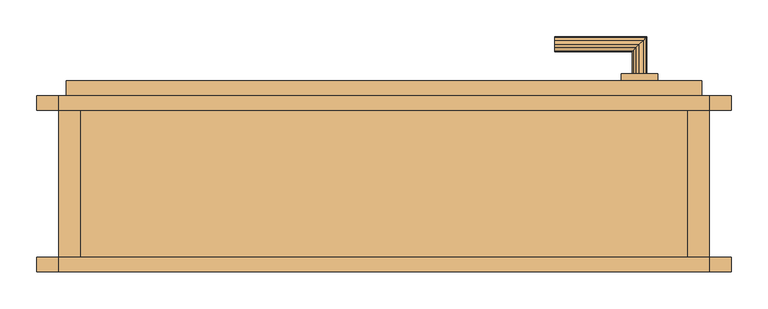
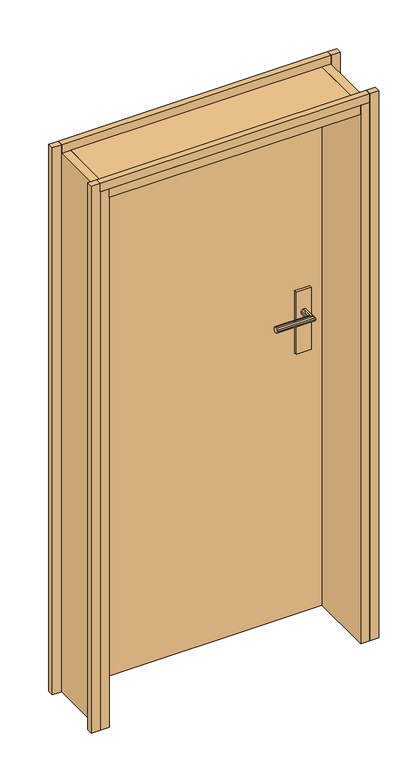
"""IFC4 building model written with IfcOpenShell, lengths in millimetres: door geometry, Tür."""

from ifc_helpers import new_model, si_unit, frame, origin, place, context, project, spatial, polyline, outline, extrude, faceted_brep, source, transform, mapped, element, save


def door_08fc6649(model_context):
    return source(origin(), model_context, "Body", "SolidModel", [
        extrude(outline(polyline([(885.0, 0.0), (885.0, -20.0), (0.0, -20.0), (0.0, 0.0), (885.0, 0.0)])), frame((0.0, 0.0, 2010.0), z_axis=(0.0, 0.0, 1.0), x_axis=(1.0, 0.0, 0.0)), (0.0, 0.0, 1.0), 30.0),
        extrude(outline(polyline([(815.0, 250.0), (815.0, 240.0), (765.0, 240.0), (765.0, 250.0), (815.0, 250.0)])), frame((0.0, 0.0, 1050.0), z_axis=(0.0, 0.0, 1.0), x_axis=(1.0, 0.0, 0.0)), (0.0, 0.0, 1.0), 215.0),
        extrude(outline(polyline([(915.0, 0.0), (915.0, -20.0), (885.0, -20.0), (885.0, 0.0), (915.0, 0.0)])), frame((0.0, 0.0, 140.0), z_axis=(0.0, 0.0, 1.0), x_axis=(1.0, 0.0, 0.0)), (0.0, 0.0, 1.0), 1900.0),
        extrude(outline(polyline([(855.0, 220.0), (855.0, -20.0), (30.0, -20.0), (30.0, 220.0), (855.0, 220.0)])), frame((0.0, 0.0, 1980.0), z_axis=(0.0, 0.0, 1.0), x_axis=(1.0, 0.0, 0.0)), (0.0, 0.0, 1.0), 30.0),
        extrude(outline(polyline([(0.0, -20.0), (-30.0, -20.0), (-30.0, 0.0), (0.0, 0.0), (0.0, -20.0)])), frame((0.0, 0.0, 140.0), z_axis=(0.0, 0.0, 1.0), x_axis=(1.0, 0.0, 0.0)), (0.0, 0.0, 1.0), 1900.0),
        extrude(outline(polyline([(765.0, 200.0), (815.0, 200.0), (815.0, 190.0), (765.0, 190.0), (765.0, 200.0)])), frame((0.0, 0.0, 1050.0), z_axis=(0.0, 0.0, 1.0), x_axis=(1.0, 0.0, 0.0)), (0.0, 0.0, 1.0), 215.0),
        extrude(outline(polyline([(885.0, 220.0), (885.0, -20.0), (855.0, -20.0), (855.0, 220.0), (885.0, 220.0)])), frame((0.0, 0.0, 140.0), z_axis=(0.0, 0.0, 1.0), x_axis=(1.0, 0.0, 0.0)), (0.0, 0.0, 1.0), 1870.0),
        faceted_brep([(795.0, 250.0, 1198.660254), (790.0, 250.0, 1200.0), (785.0, 250.0, 1198.660254), (781.339746, 250.0, 1195.0), (780.0, 250.0, 1190.0), (781.339746, 250.0, 1185.0), (785.0, 250.0, 1181.339746), (790.0, 250.0, 1180.0), (795.0, 250.0, 1181.339746), (798.660254, 250.0, 1185.0), (800.0, 250.0, 1190.0), (798.660254, 250.0, 1195.0), (790.0, 290.0, 1200.0), (795.0, 295.0, 1198.660254), (798.660254, 298.660254, 1195.0), (800.0, 300.0, 1190.0), (798.660254, 298.660254, 1185.0), (795.0, 295.0, 1181.339746), (790.0, 290.0, 1180.0), (785.0, 285.0, 1181.339746), (781.339746, 281.339746, 1185.0), (780.0, 280.0, 1190.0), (781.339746, 281.339746, 1195.0), (785.0, 285.0, 1198.660254), (675.0, 285.0, 1198.660254), (675.0, 290.0, 1200.0), (675.0, 295.0, 1198.660254), (675.0, 298.660254, 1195.0), (675.0, 300.0, 1190.0), (675.0, 298.660254, 1185.0), (675.0, 295.0, 1181.339746), (675.0, 290.0, 1180.0), (675.0, 285.0, 1181.339746), (675.0, 281.339746, 1185.0), (675.0, 280.0, 1190.0), (675.0, 281.339746, 1195.0)], [[[0, 1, 2, 3, 4, 5, 6, 7, 8, 9, 10, 11]], [[12, 1, 0, 13]], [[13, 0, 11, 14]], [[14, 11, 10, 15]], [[15, 10, 9, 16]], [[16, 9, 8, 17]], [[17, 8, 7, 18]], [[18, 7, 6, 19]], [[19, 6, 5, 20]], [[20, 5, 4, 21]], [[21, 4, 3, 22]], [[22, 3, 2, 23]], [[23, 2, 1, 12]], [[24, 25, 26, 27, 28, 29, 30, 31, 32, 33, 34, 35]], [[25, 12, 13, 26]], [[26, 13, 14, 27]], [[27, 14, 15, 28]], [[28, 15, 16, 29]], [[29, 16, 17, 30]], [[30, 17, 18, 31]], [[31, 18, 19, 32]], [[32, 19, 20, 33]], [[33, 20, 21, 34]], [[34, 21, 22, 35]], [[35, 22, 23, 24]], [[24, 23, 12, 25]]]),
        extrude(outline(polyline([(885.0, 220.0), (885.0, 200.0), (0.0, 200.0), (0.0, 220.0), (885.0, 220.0)])), frame((0.0, 0.0, 2010.0), z_axis=(0.0, 0.0, 1.0), x_axis=(1.0, 0.0, 0.0)), (0.0, 0.0, 1.0), 30.0),
        extrude(outline(polyline([(875.0, 240.0), (875.0, 200.0), (10.0, 200.0), (10.0, 240.0), (875.0, 240.0)])), frame((0.0, 0.0, 140.0), z_axis=(0.0, 0.0, 1.0), x_axis=(1.0, 0.0, 0.0)), (0.0, 0.0, 1.0), 1860.0),
        extrude(outline(polyline([(0.0, 200.0), (-30.0, 200.0), (-30.0, 220.0), (0.0, 220.0), (0.0, 200.0)])), frame((0.0, 0.0, 140.0), z_axis=(0.0, 0.0, 1.0), x_axis=(1.0, 0.0, 0.0)), (0.0, 0.0, 1.0), 1900.0),
        faceted_brep([(785.0, 190.0, 1198.660254), (790.0, 190.0, 1200.0), (795.0, 190.0, 1198.660254), (798.660254, 190.0, 1195.0), (800.0, 190.0, 1190.0), (798.660254, 190.0, 1185.0), (795.0, 190.0, 1181.339746), (790.0, 190.0, 1180.0), (785.0, 190.0, 1181.339746), (781.339746, 190.0, 1185.0), (780.0, 190.0, 1190.0), (781.339746, 190.0, 1195.0), (790.0, 150.0, 1200.0), (795.0, 145.0, 1198.660254), (798.660254, 141.339746, 1195.0), (800.0, 140.0, 1190.0), (798.660254, 141.339746, 1185.0), (795.0, 145.0, 1181.339746), (790.0, 150.0, 1180.0), (785.0, 155.0, 1181.339746), (781.339746, 158.660254, 1185.0), (780.0, 160.0, 1190.0), (781.339746, 158.660254, 1195.0), (785.0, 155.0, 1198.660254), (675.0, 145.0, 1198.660254), (675.0, 150.0, 1200.0), (675.0, 155.0, 1198.660254), (675.0, 158.660254, 1195.0), (675.0, 160.0, 1190.0), (675.0, 158.660254, 1185.0), (675.0, 155.0, 1181.339746), (675.0, 150.0, 1180.0), (675.0, 145.0, 1181.339746), (675.0, 141.339746, 1185.0), (675.0, 140.0, 1190.0), (675.0, 141.339746, 1195.0)], [[[0, 1, 2, 3, 4, 5, 6, 7, 8, 9, 10, 11]], [[2, 1, 12, 13]], [[3, 2, 13, 14]], [[4, 3, 14, 15]], [[5, 4, 15, 16]], [[6, 5, 16, 17]], [[7, 6, 17, 18]], [[8, 7, 18, 19]], [[9, 8, 19, 20]], [[10, 9, 20, 21]], [[11, 10, 21, 22]], [[0, 11, 22, 23]], [[1, 0, 23, 12]], [[24, 25, 26, 27, 28, 29, 30, 31, 32, 33, 34, 35]], [[13, 12, 25, 24]], [[14, 13, 24, 35]], [[15, 14, 35, 34]], [[16, 15, 34, 33]], [[17, 16, 33, 32]], [[18, 17, 32, 31]], [[19, 18, 31, 30]], [[20, 19, 30, 29]], [[21, 20, 29, 28]], [[22, 21, 28, 27]], [[23, 22, 27, 26]], [[12, 23, 26, 25]]]),
        extrude(outline(polyline([(915.0, 220.0), (915.0, 200.0), (885.0, 200.0), (885.0, 220.0), (915.0, 220.0)])), frame((0.0, 0.0, 140.0), z_axis=(0.0, 0.0, 1.0), x_axis=(1.0, 0.0, 0.0)), (0.0, 0.0, 1.0), 1900.0),
        extrude(outline(polyline([(30.0, 220.0), (30.0, -20.0), (0.0, -20.0), (0.0, 220.0), (30.0, 220.0)])), frame((0.0, 0.0, 140.0), z_axis=(0.0, 0.0, 1.0), x_axis=(1.0, 0.0, 0.0)), (0.0, 0.0, 1.0), 1870.0),
    ])


if __name__ == "__main__":
    model = new_model("IFC4")
    model_context = context("Model", 3, world=origin())
    ifc_project = project(units=[si_unit("LENGTHUNIT", "METRE", prefix="MILLI")], contexts=[model_context])
    site = spatial("IfcSite", under=ifc_project)
    building = spatial("IfcBuilding", under=site)
    placement = place(None, origin())
    door_shape = door_08fc6649(model_context)
    element("IfcDoor", 1, ObjectType="Tür", at=placement, inside=building, context=model_context, shape_type="MappedRepresentation", body=[
        mapped(door_shape, transform((0.0, 0.0, 0.0), x_axis=(1.0, 0.0, 0.0), y_axis=(0.0, 1.0, 0.0), z_axis=(0.0, 0.0, 1.0))),
    ])
    save(model, "model.ifc")

# Revit data of these elements
# Type "Tür"
#   Type Mark = "41"
# Element 1 (IfcDoor, "Tür")
#   Materials on its faces: "tuer_beschlag", "tuer_holzzarge"
# Materials
#   "tuer_beschlag": class "Unassigned", colour RGB 128 128 128, transparency 0
#   "tuer_holzzarge": class "Unassigned", colour RGB 255 255 255, transparency 0
